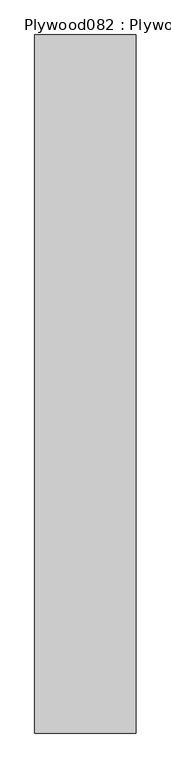
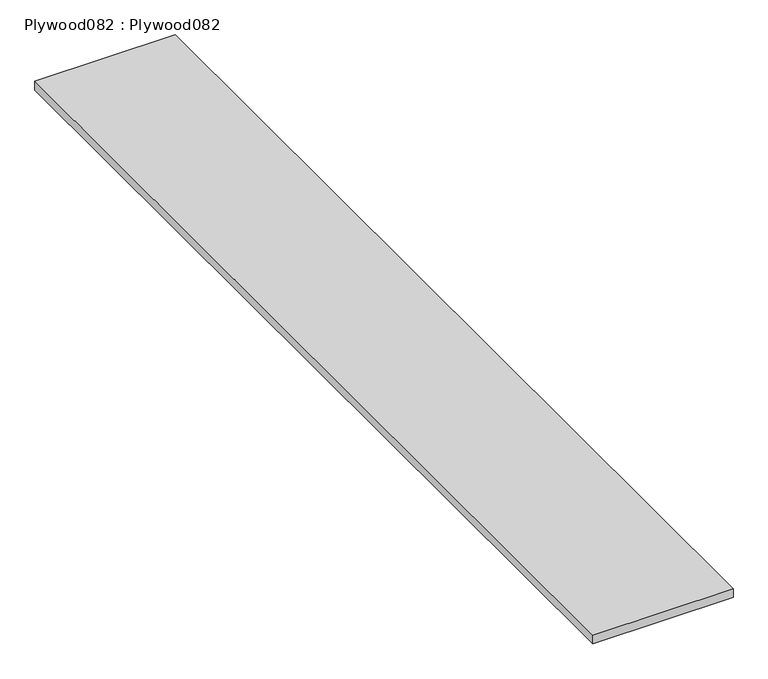
"""IFC4 building model written with IfcOpenShell, lengths in millimetres: proxy geometry, Plywood082 : Plywood082."""

import ifcopenshell
import ifcopenshell.guid

model = None  # the IFC model being written
_history = None  # IfcOwnerHistory: only IFC2X3 demands one
_inside = {}  # id of a spatial element -> (the spatial element, [elements in it])
_under = {}  # id of a project, library or spatial element -> (it, [spatial elements below it])
_declared = {}  # id of a project -> (the project, [libraries it declares])
_typed = {}  # id of a type object -> (the type object, [elements of that type])
_made_of = {}  # id of a material, layer set ... -> (it, [elements and type objects made of it])


def new_model(schema):
    """Start an empty IFC model of exactly this schema.

    Asked for "IFC4X3", IfcOpenShell would pick the latest addendum, in which some entities
    have other attributes; the version numbers below select the first issue.
    IFC2X3 requires an IfcOwnerHistory on every rooted entity: one is made here for all.
    """
    global model, _history
    if schema == "IFC4X3":
        model = ifcopenshell.file(schema_version=(4, 3, 0, 0))
    else:
        model = ifcopenshell.file(schema=schema)
    _inside.clear()
    _under.clear()
    _declared.clear()
    _typed.clear()
    _made_of.clear()
    _history = None
    if model.schema == "IFC2X3":
        org = make("IfcOrganization", Name="unknown")
        user = make(
            "IfcPersonAndOrganization",
            ThePerson=make("IfcPerson", FamilyName="unknown"),
            TheOrganization=org,
        )
        app = make(
            "IfcApplication",
            ApplicationDeveloper=org,
            Version="unknown",
            ApplicationFullName="unknown",
            ApplicationIdentifier="unknown",
        )
        _history = make(
            "IfcOwnerHistory",
            OwningUser=user,
            OwningApplication=app,
            ChangeAction="ADDED",
            CreationDate=0,
        )
    return model


def make(cls, **values):
    """One entity of the class cls with the attributes given. An attribute that is None is left unset."""
    return model.create_entity(
        cls, **{name: value for name, value in values.items() if value is not None}
    )


def rooted(cls, **values):
    """An entity with a GlobalId (a new one), such as an element, a storey or a relation."""
    return make(cls, GlobalId=ifcopenshell.guid.new(), OwnerHistory=_history, **values)


def si_unit(unit_type, name, prefix=None):
    """IfcSIUnit, for example si_unit("LENGTHUNIT", "METRE", prefix="MILLI")."""
    return make("IfcSIUnit", UnitType=unit_type, Prefix=prefix, Name=name)


def assignment(units):
    """IfcUnitAssignment: the units of a project."""
    return None if units is None else make("IfcUnitAssignment", Units=units)


def point(xyz):
    """IfcCartesianPoint."""
    return None if xyz is None else make("IfcCartesianPoint", Coordinates=xyz)


def direction(xyz):
    """IfcDirection."""
    return None if xyz is None else make("IfcDirection", DirectionRatios=xyz)


def frame(location, z_axis=None, x_axis=None):
    """IfcAxis2Placement3D, a coordinate frame: its origin and axes. An axis left out is left unset."""
    return make(
        "IfcAxis2Placement3D",
        Location=point(location),
        Axis=direction(z_axis),
        RefDirection=direction(x_axis),
    )


def origin():
    """The frame at (0, 0, 0) with its axes left unset."""
    return frame((0.0, 0.0, 0.0))


def place(relative_to, where):
    """IfcLocalPlacement: puts the frame where relative to a parent placement (None: the world)."""
    return make(
        "IfcLocalPlacement", PlacementRelTo=relative_to, RelativePlacement=where
    )


def context(
    kind, dimensions, precision=None, world=None, true_north=None, identifier=None
):
    """IfcGeometricRepresentationContext, for example the 3D "Model" context."""
    return make(
        "IfcGeometricRepresentationContext",
        ContextIdentifier=identifier,
        ContextType=kind,
        CoordinateSpaceDimension=dimensions,
        Precision=precision,
        WorldCoordinateSystem=world,
        TrueNorth=true_north,
    )


def project(units=None, contexts=None):
    """IfcProject with its units and contexts."""
    return rooted(
        "IfcProject",
        Name="project",
        RepresentationContexts=contexts,
        UnitsInContext=assignment(units),
    )


def spatial(cls, under=None, at=None, **own):
    """A site, building, storey or space (cls), placed at a placement, below another one or the project."""
    s = rooted(cls, ObjectPlacement=at, **own)
    if under is not None:
        _under.setdefault(under.id(), (under, []))[1].append(s)
    return s


def polyline(points):
    """IfcPolyline through the points."""
    return make("IfcPolyline", Points=[point(p) for p in points])


def outline(outer, holes=None, kind="AREA"):
    """IfcArbitraryClosedProfileDef: a profile drawn as a closed curve; with holes, ...WithVoids."""
    if holes is None:
        return make("IfcArbitraryClosedProfileDef", ProfileType=kind, OuterCurve=outer)
    return make(
        "IfcArbitraryProfileDefWithVoids",
        ProfileType=kind,
        OuterCurve=outer,
        InnerCurves=holes,
    )


def extrude(swept, where, along, depth):
    """IfcExtrudedAreaSolid: the profile swept, set in the frame where, extruded along a direction by depth."""
    return make(
        "IfcExtrudedAreaSolid",
        SweptArea=swept,
        Position=where,
        ExtrudedDirection=direction(along),
        Depth=depth,
    )


def shape(context_of_items, identifier, shape_type, items):
    """IfcShapeRepresentation: the items that make up one representation, for example the "Body"."""
    return make(
        "IfcShapeRepresentation",
        ContextOfItems=context_of_items,
        RepresentationIdentifier=identifier,
        RepresentationType=shape_type,
        Items=items,
    )


def source(mapping_origin, context_of_items, identifier, shape_type, items):
    """IfcRepresentationMap: a shape defined once, which mapped items show again and again."""
    return make(
        "IfcRepresentationMap",
        MappingOrigin=mapping_origin,
        MappedRepresentation=shape(context_of_items, identifier, shape_type, items),
    )


def transform(
    local_origin,
    x_axis=None,
    y_axis=None,
    z_axis=None,
    scale=None,
    scale2=None,
    scale3=None,
    uniform=True,
):
    """IfcCartesianTransformationOperator3D, or its non-uniform kind. x_axis, y_axis, z_axis: its Axis1, 2, 3."""
    if uniform:
        return make(
            "IfcCartesianTransformationOperator3D",
            Axis1=direction(x_axis),
            Axis2=direction(y_axis),
            LocalOrigin=point(local_origin),
            Scale=scale,
            Axis3=direction(z_axis),
        )
    return make(
        "IfcCartesianTransformationOperator3DnonUniform",
        Axis1=direction(x_axis),
        Axis2=direction(y_axis),
        LocalOrigin=point(local_origin),
        Scale=scale,
        Axis3=direction(z_axis),
        Scale2=scale2,
        Scale3=scale3,
    )


def mapped(mapping_source, mapping_target):
    """IfcMappedItem: shows the shape of a source again, moved by a transform."""
    return make(
        "IfcMappedItem", MappingSource=mapping_source, MappingTarget=mapping_target
    )


def made_of(thing, what):
    """Note that an element or type object is made of a material, layer set ...; save() writes the relation."""
    if what is not None:
        _made_of.setdefault(what.id(), (what, []))[1].append(thing)
    return thing


def element(
    cls,
    number,
    at=None,
    inside=None,
    cuts=None,
    type_object=None,
    material=None,
    context=None,
    identifier="Body",
    shape_type=None,
    held_by="IfcProductDefinitionShape",
    body=None,
    shapes=None,
    **own,
):
    """One element of the class cls, such as IfcWall. Its Tag is "e" and its number.

    at: its placement. inside: the storey or other place that contains it. cuts: it is an
    opening in that element (IfcRelVoidsElement). A single representation is given by context,
    identifier, shape_type and body (its items); several are given by shapes. held_by: the class
    of the entity that holds the representations. save() writes the other relations.
    """
    e = rooted(cls, Tag="e%d" % number, ObjectPlacement=at, **own)
    if body is not None:
        shapes = [shape(context, identifier, shape_type, body)]
    if shapes is not None:
        e.Representation = make(held_by, Representations=shapes)
    if inside is not None:
        _inside.setdefault(inside.id(), (inside, []))[1].append(e)
    if cuts is not None:
        rooted(
            "IfcRelVoidsElement", RelatingBuildingElement=cuts, RelatedOpeningElement=e
        )
    if type_object is not None:
        _typed.setdefault(type_object.id(), (type_object, []))[1].append(e)
    return made_of(e, material)


def aggregate(whole, parts):
    """IfcRelAggregates: a whole, such as a stair, and the parts it consists of."""
    return rooted("IfcRelAggregates", RelatingObject=whole, RelatedObjects=parts)


def save(model, path):
    """Write the relations noted so far, then the file.

    IfcRelAggregates (storeys below a building ...), IfcRelContainedInSpatialStructure (elements
    in a storey), IfcRelDefinesByType, IfcRelAssociatesMaterial and IfcRelDeclares: one each for
    every whole, place, type object, material and project.
    """
    for whole, parts in _under.values():
        aggregate(whole, parts)
    for where, things in _inside.values():
        rooted(
            "IfcRelContainedInSpatialStructure",
            RelatedElements=things,
            RelatingStructure=where,
        )
    for kind, things in _typed.values():
        rooted("IfcRelDefinesByType", RelatedObjects=things, RelatingType=kind)
    for what, things in _made_of.values():
        rooted("IfcRelAssociatesMaterial", RelatedObjects=things, RelatingMaterial=what)
    for by, libraries in _declared.values():
        rooted("IfcRelDeclares", RelatingContext=by, RelatedDefinitions=libraries)
    model.write(path)


def plywood082_plywood082_33a15e6d(model_context):
    return source(origin(), model_context, "Body", "SweptSolid", [
        extrude(outline(polyline([(-660.156476, -1052.8906574), (-950.3815411, -1052.8906574), (-950.3815411, 947.1093426), (-660.156476, 947.1093426), (-660.156476, -1052.8906574)])), frame((0.0, 0.0, 40112.696), z_axis=(0.0, 0.0, 1.0), x_axis=(1.0, 0.0, 0.0)), (0.0, 0.0, 1.0), 19.05),
    ])


if __name__ == "__main__":
    model = new_model("IFC4")
    model_context = context("Model", 3, world=origin())
    ifc_project = project(units=[si_unit("LENGTHUNIT", "METRE", prefix="MILLI")], contexts=[model_context])
    site = spatial("IfcSite", under=ifc_project)
    building = spatial("IfcBuilding", under=site)
    placement = place(None, origin())
    plywood082_plywood082_shape = plywood082_plywood082_33a15e6d(model_context)
    element("IfcBuildingElementProxy", 1, Name="Plywood082 : Plywood082", ObjectType="Plywood082 : Plywood082", at=placement, inside=building, context=model_context, shape_type="MappedRepresentation", body=[
        mapped(plywood082_plywood082_shape, transform((0.0, 0.0, 0.0), x_axis=(1.0, 0.0, 0.0), y_axis=(0.0, 1.0, 0.0), z_axis=(0.0, 0.0, 1.0))),
    ])
    save(model, "model.ifc")

# Revit data of these elements
# Type "Plywood082 : Plywood082"
#   NameOverride = "Plywood082"
# Element 1 (IfcBuildingElementProxy, "Plywood082 : Plywood082")
#   Materials on its faces: "5/8\" GYPSUM BOARD"
# Materials
#   "5/8\" GYPSUM BOARD": class "Unassigned", colour RGB 255 255 255, transparency 0, Cost = 0
